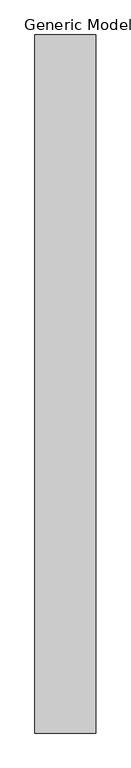
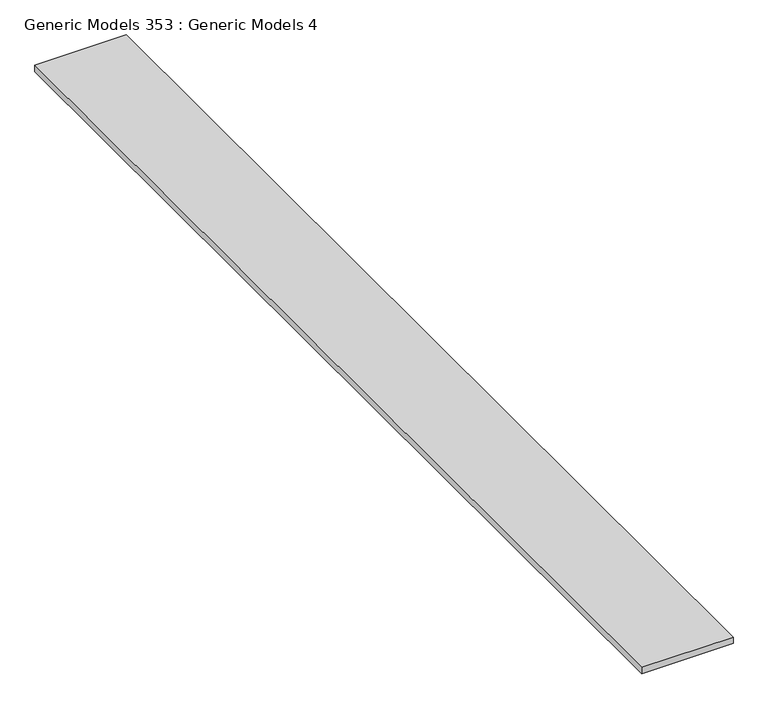
"""IFC4 building model written with IfcOpenShell, lengths in millimetres: proxy geometry, Generic Models 353 : Generic Models 4."""

from ifc_helpers import new_model, si_unit, frame, origin, place, context, project, spatial, polyline, outline, extrude, source, transform, mapped, element, save


def generic_models_353_generic_models_4_610a9001(model_context):
    return source(origin(), model_context, "Body", "SweptSolid", [
        extrude(outline(polyline([(-6410.6047749, -6864.9230338), (-6967.8925756, -6864.9230338), (-6967.8925756, -464.1230338), (-6410.6047749, -464.1230338), (-6410.6047749, -6864.9230338)])), frame((0.0, 0.0, 127277.2156), z_axis=(0.0, 0.0, 1.0), x_axis=(1.0, 0.0, 0.0)), (0.0, 0.0, 1.0), 40.9598691),
    ])


if __name__ == "__main__":
    model = new_model("IFC4")
    model_context = context("Model", 3, world=origin())
    ifc_project = project(units=[si_unit("LENGTHUNIT", "METRE", prefix="MILLI")], contexts=[model_context])
    site = spatial("IfcSite", under=ifc_project)
    building = spatial("IfcBuilding", under=site)
    placement = place(None, origin())
    generic_models_353_generic_models_4_shape = generic_models_353_generic_models_4_610a9001(model_context)
    element("IfcBuildingElementProxy", 1, Name="Generic Models 353 : Generic Models 4", ObjectType="Generic Models 353 : Generic Models 4", at=placement, inside=building, context=model_context, shape_type="MappedRepresentation", body=[
        mapped(generic_models_353_generic_models_4_shape, transform((0.0, 0.0, 0.0), x_axis=(1.0, 0.0, 0.0), y_axis=(0.0, 1.0, 0.0), z_axis=(0.0, 0.0, 1.0))),
    ])
    save(model, "model.ifc")

# Revit data of these elements
# Element 1 (IfcBuildingElementProxy, "Generic Models 353 : Generic Models 4")
#   Materials on its faces: "_BATT INSUL. (U-FACTOR = 0.065 MIN.) OVER CLASS II VAPOR RETARDER(TOWARD INTERIOR)"
# Materials
#   "_BATT INSUL. (U-FACTOR = 0.065 MIN.) OVER CLASS II VAPOR RETARDER(TOWARD INTERIOR)": class "Generic", colour RGB 200 166 247, transparency 0, Cost = 0
